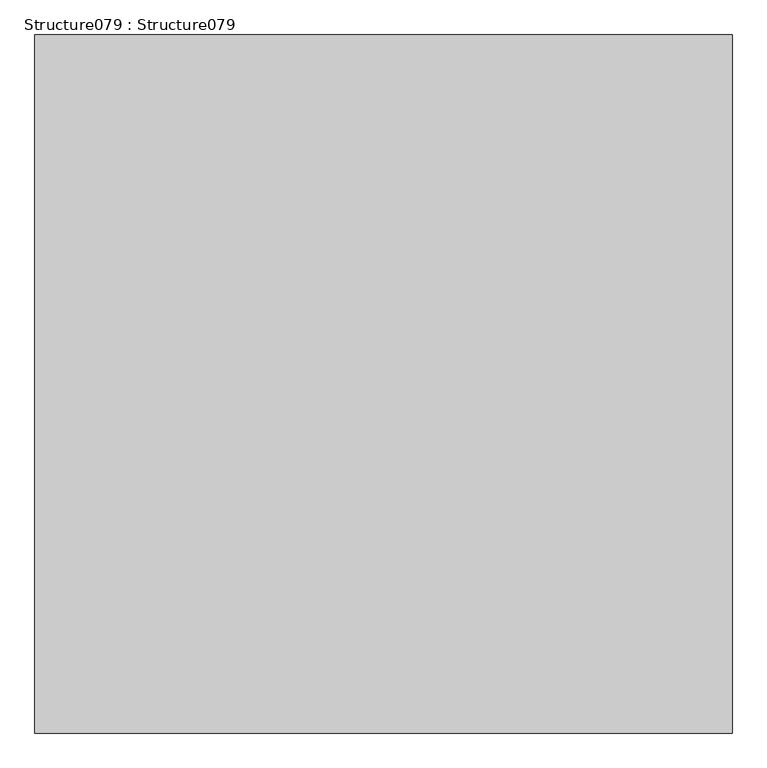
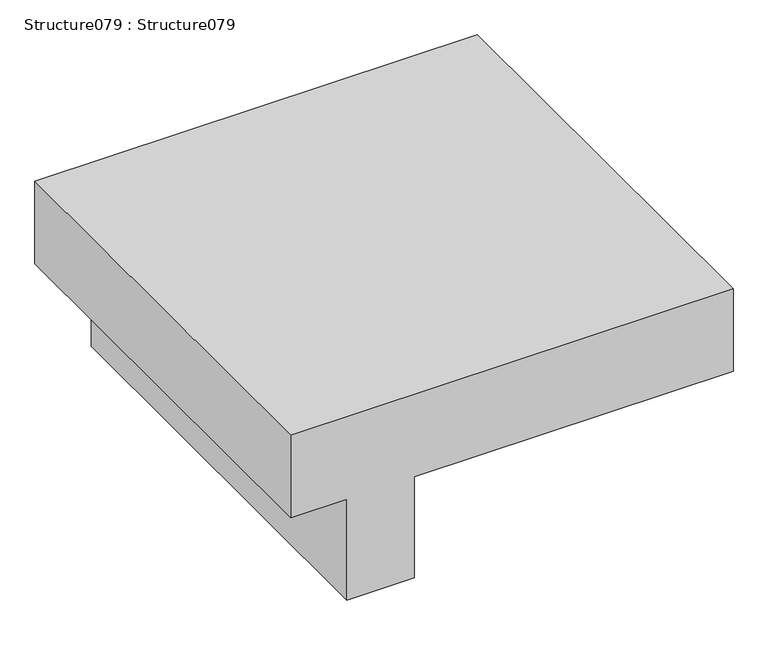
"""IFC4 building model written with IfcOpenShell, lengths in millimetres: proxy geometry, Structure079 : Structure079."""

from ifc_helpers import new_model, si_unit, frame, origin, place, context, project, spatial, polyline, outline, extrude, source, transform, mapped, element, save


def structure079_structure079_ded42bed(model_context):
    return source(origin(), model_context, "Body", "SweptSolid", [
        extrude(outline(polyline([(35667.8164062, -1544.3768494), (36150.296, -1544.3768494), (36150.296, -104.5054951), (36543.996, -104.5054951), (36543.996, -2103.1768494), (36150.296, -2103.1768494), (36150.296, -1849.1768494), (35667.8164062, -1849.1768494), (35667.8164062, -1544.3768494)])), frame((0.0, 998.1570053, 0.0), z_axis=(0.0, 1.0, 0.0), x_axis=(0.0, 0.0, 1.0)), (0.0, 0.0, 1.0), 2000.0),
    ])


if __name__ == "__main__":
    model = new_model("IFC4")
    model_context = context("Model", 3, world=origin())
    ifc_project = project(units=[si_unit("LENGTHUNIT", "METRE", prefix="MILLI")], contexts=[model_context])
    site = spatial("IfcSite", under=ifc_project)
    building = spatial("IfcBuilding", under=site)
    placement = place(None, origin())
    structure079_structure079_shape = structure079_structure079_ded42bed(model_context)
    element("IfcBuildingElementProxy", 1, Name="Structure079 : Structure079", ObjectType="Structure079 : Structure079", at=placement, inside=building, context=model_context, shape_type="MappedRepresentation", body=[
        mapped(structure079_structure079_shape, transform((0.0, 0.0, 0.0), x_axis=(1.0, 0.0, 0.0), y_axis=(0.0, 1.0, 0.0), z_axis=(0.0, 0.0, 1.0))),
    ])
    save(model, "model.ifc")

# Revit data of these elements
# Type "Structure079 : Structure079"
#   NameOverride = "Structure079"
# Element 1 (IfcBuildingElementProxy, "Structure079 : Structure079")
#   Materials on its faces: "CONCRETE SLAB W/ GRADE BEAM (SEE STRUCT DWGS)"
# Materials
#   "CONCRETE SLAB W/ GRADE BEAM (SEE STRUCT DWGS)": class "Unassigned", colour RGB 128 128 128, transparency 0, Cost = 0
